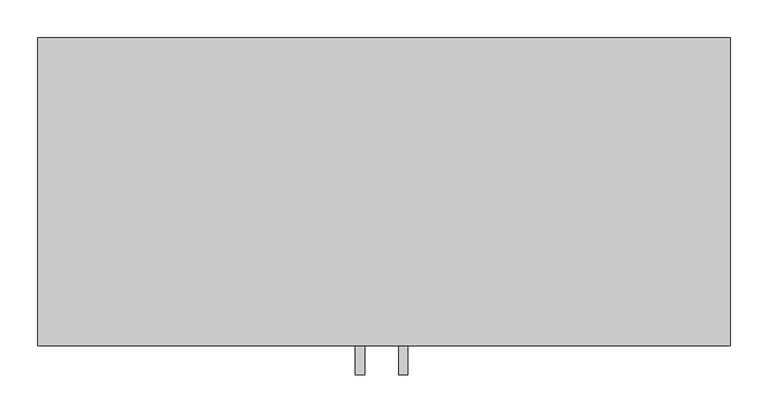
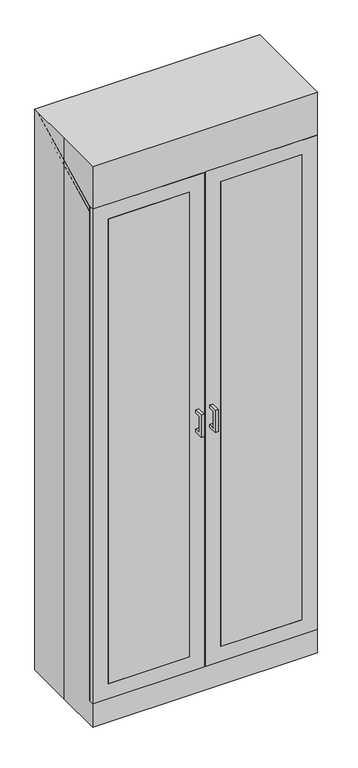
"""IFC4 building model written with IfcOpenShell, lengths in millimetres: proxy geometry, CW090 - Cabinet, Floor Standing, 5 SH, 2 GDO, ST, 95x36x16 : CW090 - Cabinet, Floor Standing, 5 SH, 2 GDO, ST, 95x36x16."""

import ifcopenshell
import ifcopenshell.guid

model = None  # the IFC model being written
_history = None  # IfcOwnerHistory: only IFC2X3 demands one
_inside = {}  # id of a spatial element -> (the spatial element, [elements in it])
_under = {}  # id of a project, library or spatial element -> (it, [spatial elements below it])
_declared = {}  # id of a project -> (the project, [libraries it declares])
_typed = {}  # id of a type object -> (the type object, [elements of that type])
_made_of = {}  # id of a material, layer set ... -> (it, [elements and type objects made of it])


def new_model(schema):
    """Start an empty IFC model of exactly this schema.

    Asked for "IFC4X3", IfcOpenShell would pick the latest addendum, in which some entities
    have other attributes; the version numbers below select the first issue.
    IFC2X3 requires an IfcOwnerHistory on every rooted entity: one is made here for all.
    """
    global model, _history
    if schema == "IFC4X3":
        model = ifcopenshell.file(schema_version=(4, 3, 0, 0))
    else:
        model = ifcopenshell.file(schema=schema)
    _inside.clear()
    _under.clear()
    _declared.clear()
    _typed.clear()
    _made_of.clear()
    _history = None
    if model.schema == "IFC2X3":
        org = make("IfcOrganization", Name="unknown")
        user = make(
            "IfcPersonAndOrganization",
            ThePerson=make("IfcPerson", FamilyName="unknown"),
            TheOrganization=org,
        )
        app = make(
            "IfcApplication",
            ApplicationDeveloper=org,
            Version="unknown",
            ApplicationFullName="unknown",
            ApplicationIdentifier="unknown",
        )
        _history = make(
            "IfcOwnerHistory",
            OwningUser=user,
            OwningApplication=app,
            ChangeAction="ADDED",
            CreationDate=0,
        )
    return model


def make(cls, **values):
    """One entity of the class cls with the attributes given. An attribute that is None is left unset."""
    return model.create_entity(
        cls, **{name: value for name, value in values.items() if value is not None}
    )


def rooted(cls, **values):
    """An entity with a GlobalId (a new one), such as an element, a storey or a relation."""
    return make(cls, GlobalId=ifcopenshell.guid.new(), OwnerHistory=_history, **values)


def si_unit(unit_type, name, prefix=None):
    """IfcSIUnit, for example si_unit("LENGTHUNIT", "METRE", prefix="MILLI")."""
    return make("IfcSIUnit", UnitType=unit_type, Prefix=prefix, Name=name)


def assignment(units):
    """IfcUnitAssignment: the units of a project."""
    return None if units is None else make("IfcUnitAssignment", Units=units)


def point(xyz):
    """IfcCartesianPoint."""
    return None if xyz is None else make("IfcCartesianPoint", Coordinates=xyz)


def direction(xyz):
    """IfcDirection."""
    return None if xyz is None else make("IfcDirection", DirectionRatios=xyz)


def frame(location, z_axis=None, x_axis=None):
    """IfcAxis2Placement3D, a coordinate frame: its origin and axes. An axis left out is left unset."""
    return make(
        "IfcAxis2Placement3D",
        Location=point(location),
        Axis=direction(z_axis),
        RefDirection=direction(x_axis),
    )


def origin():
    """The frame at (0, 0, 0) with its axes left unset."""
    return frame((0.0, 0.0, 0.0))


def origin_with_axes():
    """The frame at (0, 0, 0) with the z axis (0, 0, 1) and the x axis (1, 0, 0) written out."""
    return frame((0.0, 0.0, 0.0), z_axis=(0.0, 0.0, 1.0), x_axis=(1.0, 0.0, 0.0))


def place(relative_to, where):
    """IfcLocalPlacement: puts the frame where relative to a parent placement (None: the world)."""
    return make(
        "IfcLocalPlacement", PlacementRelTo=relative_to, RelativePlacement=where
    )


def context(
    kind, dimensions, precision=None, world=None, true_north=None, identifier=None
):
    """IfcGeometricRepresentationContext, for example the 3D "Model" context."""
    return make(
        "IfcGeometricRepresentationContext",
        ContextIdentifier=identifier,
        ContextType=kind,
        CoordinateSpaceDimension=dimensions,
        Precision=precision,
        WorldCoordinateSystem=world,
        TrueNorth=true_north,
    )


def project(units=None, contexts=None):
    """IfcProject with its units and contexts."""
    return rooted(
        "IfcProject",
        Name="project",
        RepresentationContexts=contexts,
        UnitsInContext=assignment(units),
    )


def spatial(cls, under=None, at=None, **own):
    """A site, building, storey or space (cls), placed at a placement, below another one or the project."""
    s = rooted(cls, ObjectPlacement=at, **own)
    if under is not None:
        _under.setdefault(under.id(), (under, []))[1].append(s)
    return s


def polyline(points):
    """IfcPolyline through the points."""
    return make("IfcPolyline", Points=[point(p) for p in points])


def outline(outer, holes=None, kind="AREA"):
    """IfcArbitraryClosedProfileDef: a profile drawn as a closed curve; with holes, ...WithVoids."""
    if holes is None:
        return make("IfcArbitraryClosedProfileDef", ProfileType=kind, OuterCurve=outer)
    return make(
        "IfcArbitraryProfileDefWithVoids",
        ProfileType=kind,
        OuterCurve=outer,
        InnerCurves=holes,
    )


def extrude(swept, where, along, depth):
    """IfcExtrudedAreaSolid: the profile swept, set in the frame where, extruded along a direction by depth."""
    return make(
        "IfcExtrudedAreaSolid",
        SweptArea=swept,
        Position=where,
        ExtrudedDirection=direction(along),
        Depth=depth,
    )


def faces_of(points, faces, orient=None, outer=None):
    """IfcFace entities. A face is a list of loops; a loop is a list of indices into points, from 0.

    orient and outer hold one flag for each loop. By default every Orientation is true, the
    first loop of a face is its IfcFaceOuterBound and the others are IfcFaceBound.
    """
    made = []
    for i, loops in enumerate(faces):
        bounds = []
        for j, loop in enumerate(loops):
            is_outer = j == 0 if outer is None else outer[i][j]
            bounds.append(
                make(
                    "IfcFaceOuterBound" if is_outer else "IfcFaceBound",
                    Bound=make("IfcPolyLoop", Polygon=[points[k] for k in loop]),
                    Orientation=True if orient is None else orient[i][j],
                )
            )
        made.append(make("IfcFace", Bounds=bounds))
    return made


def faceted_brep(points, faces, orient=None, outer=None, voids=None):
    """IfcFacetedBrep: a solid bounded by flat faces; with voids (closed shells), ...WithVoids."""
    shared = [point(p) for p in points]
    hull = make("IfcClosedShell", CfsFaces=faces_of(shared, faces, orient, outer))
    if voids is None:
        return make("IfcFacetedBrep", Outer=hull)
    return make(
        "IfcFacetedBrepWithVoids",
        Outer=hull,
        Voids=[
            make(cls, CfsFaces=faces_of(shared, fs, o, b)) for cls, fs, o, b in voids
        ],
    )


def shape(context_of_items, identifier, shape_type, items):
    """IfcShapeRepresentation: the items that make up one representation, for example the "Body"."""
    return make(
        "IfcShapeRepresentation",
        ContextOfItems=context_of_items,
        RepresentationIdentifier=identifier,
        RepresentationType=shape_type,
        Items=items,
    )


def source(mapping_origin, context_of_items, identifier, shape_type, items):
    """IfcRepresentationMap: a shape defined once, which mapped items show again and again."""
    return make(
        "IfcRepresentationMap",
        MappingOrigin=mapping_origin,
        MappedRepresentation=shape(context_of_items, identifier, shape_type, items),
    )


def transform(
    local_origin,
    x_axis=None,
    y_axis=None,
    z_axis=None,
    scale=None,
    scale2=None,
    scale3=None,
    uniform=True,
):
    """IfcCartesianTransformationOperator3D, or its non-uniform kind. x_axis, y_axis, z_axis: its Axis1, 2, 3."""
    if uniform:
        return make(
            "IfcCartesianTransformationOperator3D",
            Axis1=direction(x_axis),
            Axis2=direction(y_axis),
            LocalOrigin=point(local_origin),
            Scale=scale,
            Axis3=direction(z_axis),
        )
    return make(
        "IfcCartesianTransformationOperator3DnonUniform",
        Axis1=direction(x_axis),
        Axis2=direction(y_axis),
        LocalOrigin=point(local_origin),
        Scale=scale,
        Axis3=direction(z_axis),
        Scale2=scale2,
        Scale3=scale3,
    )


def mapped(mapping_source, mapping_target):
    """IfcMappedItem: shows the shape of a source again, moved by a transform."""
    return make(
        "IfcMappedItem", MappingSource=mapping_source, MappingTarget=mapping_target
    )


def made_of(thing, what):
    """Note that an element or type object is made of a material, layer set ...; save() writes the relation."""
    if what is not None:
        _made_of.setdefault(what.id(), (what, []))[1].append(thing)
    return thing


def element(
    cls,
    number,
    at=None,
    inside=None,
    cuts=None,
    type_object=None,
    material=None,
    context=None,
    identifier="Body",
    shape_type=None,
    held_by="IfcProductDefinitionShape",
    body=None,
    shapes=None,
    **own,
):
    """One element of the class cls, such as IfcWall. Its Tag is "e" and its number.

    at: its placement. inside: the storey or other place that contains it. cuts: it is an
    opening in that element (IfcRelVoidsElement). A single representation is given by context,
    identifier, shape_type and body (its items); several are given by shapes. held_by: the class
    of the entity that holds the representations. save() writes the other relations.
    """
    e = rooted(cls, Tag="e%d" % number, ObjectPlacement=at, **own)
    if body is not None:
        shapes = [shape(context, identifier, shape_type, body)]
    if shapes is not None:
        e.Representation = make(held_by, Representations=shapes)
    if inside is not None:
        _inside.setdefault(inside.id(), (inside, []))[1].append(e)
    if cuts is not None:
        rooted(
            "IfcRelVoidsElement", RelatingBuildingElement=cuts, RelatedOpeningElement=e
        )
    if type_object is not None:
        _typed.setdefault(type_object.id(), (type_object, []))[1].append(e)
    return made_of(e, material)


def aggregate(whole, parts):
    """IfcRelAggregates: a whole, such as a stair, and the parts it consists of."""
    return rooted("IfcRelAggregates", RelatingObject=whole, RelatedObjects=parts)


def save(model, path):
    """Write the relations noted so far, then the file.

    IfcRelAggregates (storeys below a building ...), IfcRelContainedInSpatialStructure (elements
    in a storey), IfcRelDefinesByType, IfcRelAssociatesMaterial and IfcRelDeclares: one each for
    every whole, place, type object, material and project.
    """
    for whole, parts in _under.values():
        aggregate(whole, parts)
    for where, things in _inside.values():
        rooted(
            "IfcRelContainedInSpatialStructure",
            RelatedElements=things,
            RelatingStructure=where,
        )
    for kind, things in _typed.values():
        rooted("IfcRelDefinesByType", RelatedObjects=things, RelatingType=kind)
    for what, things in _made_of.values():
        rooted("IfcRelAssociatesMaterial", RelatedObjects=things, RelatingMaterial=what)
    for by, libraries in _declared.values():
        rooted("IfcRelDeclares", RelatingContext=by, RelatedDefinitions=libraries)
    model.write(path)


def specialty_equipment_72b9e3d9(model_context):
    return source(origin(), model_context, "Body", "SolidModel", [
        extrude(outline(polyline([(-63.5, -203.2), (-393.7, -203.2), (-393.7, -196.85), (-63.5, -196.85), (-63.5, -203.2)])), frame((0.0, 0.0, 165.1), z_axis=(0.0, 0.0, 1.0), x_axis=(1.0, 0.0, 0.0)), (0.0, 0.0, 1.0), 2000.25),
        extrude(outline(polyline([(-241.2716405, 1219.2), (-203.1905468, 1219.2), (-203.1905468, 1206.5303499), (-228.6019905, 1206.5303499), (-228.6019905, 1136.6574627), (-203.1905468, 1136.6574627), (-203.1905468, 1123.9878126), (-241.2716405, 1123.9878126), (-241.2716405, 1219.2)])), frame((-37.9511719, 0.0, 0.0), z_axis=(1.0, 0.0, 0.0), x_axis=(0.0, 1.0, 0.0)), (0.0, 0.0, 1.0), 12.4023438),
        extrude(outline(polyline([(-241.2716405, 1219.2), (-203.1905468, 1219.2), (-203.1905468, 1206.5303499), (-228.6019905, 1206.5303499), (-228.6019905, 1136.6574627), (-203.1905468, 1136.6574627), (-203.1905468, 1123.9878126), (-241.2716405, 1123.9878126), (-241.2716405, 1219.2)])), frame((19.1988281, 0.0, 0.0), z_axis=(1.0, 0.0, 0.0), x_axis=(0.0, 1.0, 0.0)), (0.0, 0.0, 1.0), 12.4023437),
        extrude(outline(polyline([(2228.85, -457.2), (101.6, -457.2), (101.6, -3.175), (2228.85, -3.175), (2228.85, -457.2)]), holes=[polyline([(165.1, -393.7), (2165.35, -393.7), (2165.35, -63.5), (165.1, -63.5), (165.1, -393.7)])]), frame((0.0, -203.2, 0.0), z_axis=(0.0, 1.0, 0.0), x_axis=(0.0, 0.0, 1.0)), (0.0, 0.0, 1.0), 19.05),
        extrude(outline(polyline([(393.7, -203.2), (63.5, -203.2), (63.5, -196.85), (393.7, -196.85), (393.7, -203.2)])), frame((0.0, 0.0, 165.1), z_axis=(0.0, 0.0, 1.0), x_axis=(1.0, 0.0, 0.0)), (0.0, 0.0, 1.0), 2000.25),
        extrude(outline(polyline([(2228.85, 457.2), (2228.85, 3.175), (101.6, 3.175), (101.6, 457.2), (2228.85, 457.2)]), holes=[polyline([(2165.35, 393.7), (165.1, 393.7), (165.1, 63.5), (2165.35, 63.5), (2165.35, 393.7)])]), frame((0.0, -203.2, 0.0), z_axis=(0.0, 1.0, 0.0), x_axis=(0.0, 0.0, 1.0)), (0.0, 0.0, 1.0), 19.05),
        extrude(outline(polyline([(438.15, -184.15), (-438.15, -184.15), (-438.15, 184.15), (438.15, 184.15), (438.15, -184.15)])), frame((0.0, 0.0, 1473.2), z_axis=(0.0, 0.0, 1.0), x_axis=(1.0, 0.0, 0.0)), (0.0, 0.0, 1.0), 25.4),
        extrude(outline(polyline([(438.15, -184.15), (-438.15, -184.15), (-438.15, 184.15), (438.15, 184.15), (438.15, -184.15)])), frame((0.0, 0.0, 1854.2), z_axis=(0.0, 0.0, 1.0), x_axis=(1.0, 0.0, 0.0)), (0.0, 0.0, 1.0), 25.4),
        extrude(outline(polyline([(438.15, -184.15), (-438.15, -184.15), (-438.15, 184.15), (438.15, 184.15), (438.15, -184.15)])), frame((0.0, 0.0, 1117.6), z_axis=(0.0, 0.0, 1.0), x_axis=(1.0, 0.0, 0.0)), (0.0, 0.0, 1.0), 25.4),
        extrude(outline(polyline([(438.15, -184.15), (-438.15, -184.15), (-438.15, 184.15), (438.15, 184.15), (438.15, -184.15)])), frame((0.0, 0.0, 787.4), z_axis=(0.0, 0.0, 1.0), x_axis=(1.0, 0.0, 0.0)), (0.0, 0.0, 1.0), 25.4),
        extrude(outline(polyline([(438.15, -184.15), (-438.15, -184.15), (-438.15, 184.15), (438.15, 184.15), (438.15, -184.15)])), frame((0.0, 0.0, 419.1), z_axis=(0.0, 0.0, 1.0), x_axis=(1.0, 0.0, 0.0)), (0.0, 0.0, 1.0), 25.4),
        faceted_brep([(-457.2, 203.2, 2413.0), (-457.2, 0.0, 2413.0), (-457.2, -203.2, 2413.0), (457.2, -203.2, 2413.0), (457.2, 203.2, 2413.0), (-457.2, 203.2, 0.0), (457.2, 203.2, 0.0), (457.2, -203.2, 0.0), (-457.2, -203.2, 0.0), (-457.2, 0.0, 0.0), (393.7, -203.2, 2165.35), (393.7, -203.2, 165.1), (63.5, -203.2, 165.1), (63.5, -203.2, 2165.35), (-393.7, -203.2, 165.1), (-393.7, -203.2, 2165.35), (-63.5, -203.2, 2165.35), (-63.5, -203.2, 165.1), (393.7, -184.15, 2165.35), (393.7, -184.15, 165.1), (63.5, -184.15, 2165.35), (63.5, -184.15, 165.1), (-393.7, -184.15, 2165.35), (-393.7, -184.15, 165.1), (-63.5, -184.15, 2165.35), (-63.5, -184.15, 165.1)], [[[0, 1, 2, 3, 4]], [[5, 6, 7, 8, 9]], [[1, 0, 5, 9]], [[2, 1, 9, 8]], [[3, 2, 8, 7], [10, 11, 12, 13], [14, 15, 16, 17]], [[4, 3, 7, 6]], [[0, 4, 6, 5]], [[18, 19, 11, 10]], [[20, 13, 12, 21]], [[18, 10, 13, 20]], [[11, 19, 21, 12]], [[19, 18, 20, 21]], [[22, 15, 14, 23]], [[24, 25, 17, 16]], [[15, 22, 24, 16]], [[23, 14, 17, 25]], [[22, 23, 25, 24]]]),
        extrude(outline(polyline([(184.15, 2391.7014525), (184.15, 101.6), (-184.15, 101.6), (-184.15, 2207.5514525), (184.15, 2391.7014525)])), frame((-457.2, 0.0, 0.0), z_axis=(1.0, 0.0, 0.0), x_axis=(0.0, 1.0, 0.0)), (0.0, 0.0, 1.0), 19.05),
        extrude(outline(polyline([(184.15, 2391.7014525), (184.15, 101.6), (-184.15, 101.6), (-184.15, 2207.5514525), (184.15, 2391.7014525)])), frame((438.15, 0.0, 0.0), z_axis=(1.0, 0.0, 0.0), x_axis=(0.0, 1.0, 0.0)), (0.0, 0.0, 1.0), 19.05),
        extrude(outline(polyline([(-438.15, 184.15), (-438.15, -127.0), (-457.2, -127.0), (-457.2, 184.15), (-438.15, 184.15)])), origin_with_axes(), (0.0, 0.0, 1.0), 101.6),
        extrude(outline(polyline([(457.2, 184.15), (457.2, -127.0), (438.15, -127.0), (438.15, 184.15), (457.2, 184.15)])), origin_with_axes(), (0.0, 0.0, 1.0), 101.6),
        extrude(outline(polyline([(-184.15, 2228.85), (184.15, 2413.0), (184.15, 2391.7014525), (-184.15, 2207.5514525), (-184.15, 2228.85)])), frame((-457.2, 0.0, 0.0), z_axis=(1.0, 0.0, 0.0), x_axis=(0.0, 1.0, 0.0)), (0.0, 0.0, 1.0), 914.4),
        extrude(outline(polyline([(438.15, -184.15), (-438.15, -184.15), (-438.15, 184.15), (438.15, 184.15), (438.15, -184.15)])), frame((0.0, 0.0, 101.6), z_axis=(0.0, 0.0, 1.0), x_axis=(1.0, 0.0, 0.0)), (0.0, 0.0, 1.0), 25.4),
        extrude(outline(polyline([(457.2, -107.95), (457.2, -127.0), (-457.2, -127.0), (-457.2, -107.95), (457.2, -107.95)])), origin_with_axes(), (0.0, 0.0, 1.0), 101.6),
        extrude(outline(polyline([(457.2, 184.15), (-457.2, 184.15), (-457.2, 203.2), (457.2, 203.2), (457.2, 184.15)])), origin_with_axes(), (0.0, 0.0, 1.0), 2413.0),
    ])


if __name__ == "__main__":
    model = new_model("IFC4")
    model_context = context("Model", 3, world=origin())
    ifc_project = project(units=[si_unit("LENGTHUNIT", "METRE", prefix="MILLI")], contexts=[model_context])
    site = spatial("IfcSite", under=ifc_project)
    building = spatial("IfcBuilding", under=site)
    placement = place(None, origin())
    specialty_equipment_shape = specialty_equipment_72b9e3d9(model_context)
    element("IfcBuildingElementProxy", 1, Name="CW090 - Cabinet, Floor Standing, 5 SH, 2 GDO, ST, 95x36x16 : CW090 - Cabinet, Floor Standing, 5 SH, 2 GDO, ST, 95x36x16", ObjectType="CW090 - Cabinet, Floor Standing, 5 SH, 2 GDO, ST, 95x36x16 : CW090 - Cabinet, Floor Standing, 5 SH, 2 GDO, ST, 95x36x16", at=placement, inside=building, context=model_context, shape_type="MappedRepresentation", body=[
        mapped(specialty_equipment_shape, transform((0.0, 0.0, 0.0), x_axis=(1.0, 0.0, 0.0), y_axis=(0.0, 1.0, 0.0), z_axis=(0.0, 0.0, 1.0))),
    ])
    save(model, "model.ifc")

# Revit data of these elements
# Project information
#   Room Abbreviation = "VNEC1"
#   Room Description = "Necropsy, Veterinary (VNEC1)"
#   Sheets - Total = "5"
#   Project Issue Date = "Issue Date"
#   Project Status = "Project Status"
#   Client Name = "Owner"
#   Project Address = "Enter address here"
#   Project Name = "Project Name"
#   Project Number = "Project Number"
#   Publication Date = "1-Feb-16"
# Type "CW090 - Cabinet, Floor Standing, 5 SH, 2 GDO, ST, 95x36x16 : CW090 - Cabinet, Floor Standing, 5 SH, 2 GDO, ST, 95x36x16"
#   Watts2 = "0"
#   Watts1 = "0"
#   Unit_Issue = "EA"
#   UTIL_6_Misc = "-"
#   UTIL_5_NonMedGas = "-"
#   UTIL_4_MiscGas = "-"
#   UTIL_3_MedGas = "-"
#   UTIL_2_Elec = "-"
#   UTIL_1_WaterDrain = "-"
#   Nomenclature = "Cabinet, Floor Standing, 5 SH, 2 GDO, ST, 95\"x36\""
#   NSN = "6530"
#   Location [instance default] = ""
#   JSN = "CW090"
#   Fund_Source_VA = "-"
#   Fund_Source_Navy = "-"
#   Fund_Source_Army = "-"
#   Fund_Source_AF = "-"
#   ELEC_Volts2 = "0"
#   ELEC_Volts1 = "0"
#   ELEC_Phase2 = "0"
#   ELEC_Phase1 = "0"
#   ELEC_HertzSwitch = "0"
#   ELEC_HertzDependent = "0"
#   ELEC_Hertz = "0"
#   ELEC_Amps2 = "0"
#   ELEC_Amps1 = "0"
#   DetailDescription = "Floor standing storage cabinet approximately 95\" H x 36\" W x 16\" D with five adjustable shelves, framed glass hinged doors, and sloping top. Also referred to as a framed glass hinged double door case. For general purpose use throughout the facility."
#   CAT_VA = "A"
#   CAT_Navy = "A"
#   CAT_IHS = "-"
#   CAT_Army = "A"
#   CAT_AF = "A"
#   BTUperhour = "0"
#   Weight_IP = 293
#   DIM_Width_IP = 3' - 0"
#   DIM_Height_IP = 7' - 11"
#   DIM_Depth_IP = 1' - 4"
# Element 1 (IfcBuildingElementProxy, "CW090 - Cabinet, Floor Standing, 5 SH, 2 GDO, ST, 95x36x16 : CW090 - Cabinet, Floor Standing, 5 SH, 2 GDO, ST, 95x36x16")
#   Materials on its faces: "Default metal", "EquipSpace", "Glass"
# Materials
#   "Default metal": class "Unassigned", colour RGB 204 204 204, transparency 0
#   "EquipSpace": class "Unassigned", colour RGB 221 217 195, transparency 0.5
#   "Glass": class "Glass", colour RGB 0 128 192, transparency 0.75
